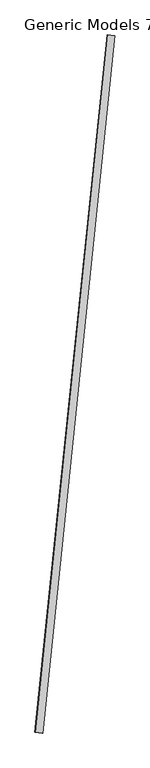
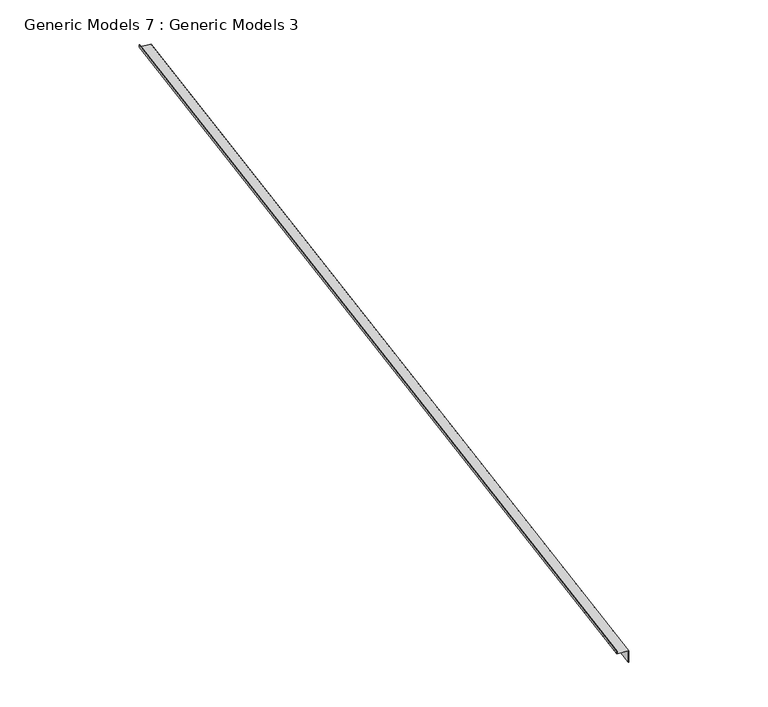
"""IFC4 building model written with IfcOpenShell, lengths in millimetres: proxy geometry, Generic Models 7 : Generic Models 3."""

import ifcopenshell
import ifcopenshell.guid

model = None  # the IFC model being written
_history = None  # IfcOwnerHistory: only IFC2X3 demands one
_inside = {}  # id of a spatial element -> (the spatial element, [elements in it])
_under = {}  # id of a project, library or spatial element -> (it, [spatial elements below it])
_declared = {}  # id of a project -> (the project, [libraries it declares])
_typed = {}  # id of a type object -> (the type object, [elements of that type])
_made_of = {}  # id of a material, layer set ... -> (it, [elements and type objects made of it])


def new_model(schema):
    """Start an empty IFC model of exactly this schema.

    Asked for "IFC4X3", IfcOpenShell would pick the latest addendum, in which some entities
    have other attributes; the version numbers below select the first issue.
    IFC2X3 requires an IfcOwnerHistory on every rooted entity: one is made here for all.
    """
    global model, _history
    if schema == "IFC4X3":
        model = ifcopenshell.file(schema_version=(4, 3, 0, 0))
    else:
        model = ifcopenshell.file(schema=schema)
    _inside.clear()
    _under.clear()
    _declared.clear()
    _typed.clear()
    _made_of.clear()
    _history = None
    if model.schema == "IFC2X3":
        org = make("IfcOrganization", Name="unknown")
        user = make(
            "IfcPersonAndOrganization",
            ThePerson=make("IfcPerson", FamilyName="unknown"),
            TheOrganization=org,
        )
        app = make(
            "IfcApplication",
            ApplicationDeveloper=org,
            Version="unknown",
            ApplicationFullName="unknown",
            ApplicationIdentifier="unknown",
        )
        _history = make(
            "IfcOwnerHistory",
            OwningUser=user,
            OwningApplication=app,
            ChangeAction="ADDED",
            CreationDate=0,
        )
    return model


def make(cls, **values):
    """One entity of the class cls with the attributes given. An attribute that is None is left unset."""
    return model.create_entity(
        cls, **{name: value for name, value in values.items() if value is not None}
    )


def rooted(cls, **values):
    """An entity with a GlobalId (a new one), such as an element, a storey or a relation."""
    return make(cls, GlobalId=ifcopenshell.guid.new(), OwnerHistory=_history, **values)


def si_unit(unit_type, name, prefix=None):
    """IfcSIUnit, for example si_unit("LENGTHUNIT", "METRE", prefix="MILLI")."""
    return make("IfcSIUnit", UnitType=unit_type, Prefix=prefix, Name=name)


def assignment(units):
    """IfcUnitAssignment: the units of a project."""
    return None if units is None else make("IfcUnitAssignment", Units=units)


def point(xyz):
    """IfcCartesianPoint."""
    return None if xyz is None else make("IfcCartesianPoint", Coordinates=xyz)


def direction(xyz):
    """IfcDirection."""
    return None if xyz is None else make("IfcDirection", DirectionRatios=xyz)


def frame(location, z_axis=None, x_axis=None):
    """IfcAxis2Placement3D, a coordinate frame: its origin and axes. An axis left out is left unset."""
    return make(
        "IfcAxis2Placement3D",
        Location=point(location),
        Axis=direction(z_axis),
        RefDirection=direction(x_axis),
    )


def origin():
    """The frame at (0, 0, 0) with its axes left unset."""
    return frame((0.0, 0.0, 0.0))


def place(relative_to, where):
    """IfcLocalPlacement: puts the frame where relative to a parent placement (None: the world)."""
    return make(
        "IfcLocalPlacement", PlacementRelTo=relative_to, RelativePlacement=where
    )


def context(
    kind, dimensions, precision=None, world=None, true_north=None, identifier=None
):
    """IfcGeometricRepresentationContext, for example the 3D "Model" context."""
    return make(
        "IfcGeometricRepresentationContext",
        ContextIdentifier=identifier,
        ContextType=kind,
        CoordinateSpaceDimension=dimensions,
        Precision=precision,
        WorldCoordinateSystem=world,
        TrueNorth=true_north,
    )


def project(units=None, contexts=None):
    """IfcProject with its units and contexts."""
    return rooted(
        "IfcProject",
        Name="project",
        RepresentationContexts=contexts,
        UnitsInContext=assignment(units),
    )


def spatial(cls, under=None, at=None, **own):
    """A site, building, storey or space (cls), placed at a placement, below another one or the project."""
    s = rooted(cls, ObjectPlacement=at, **own)
    if under is not None:
        _under.setdefault(under.id(), (under, []))[1].append(s)
    return s


def polyline(points):
    """IfcPolyline through the points."""
    return make("IfcPolyline", Points=[point(p) for p in points])


def outline(outer, holes=None, kind="AREA"):
    """IfcArbitraryClosedProfileDef: a profile drawn as a closed curve; with holes, ...WithVoids."""
    if holes is None:
        return make("IfcArbitraryClosedProfileDef", ProfileType=kind, OuterCurve=outer)
    return make(
        "IfcArbitraryProfileDefWithVoids",
        ProfileType=kind,
        OuterCurve=outer,
        InnerCurves=holes,
    )


def extrude(swept, where, along, depth):
    """IfcExtrudedAreaSolid: the profile swept, set in the frame where, extruded along a direction by depth."""
    return make(
        "IfcExtrudedAreaSolid",
        SweptArea=swept,
        Position=where,
        ExtrudedDirection=direction(along),
        Depth=depth,
    )


def shape(context_of_items, identifier, shape_type, items):
    """IfcShapeRepresentation: the items that make up one representation, for example the "Body"."""
    return make(
        "IfcShapeRepresentation",
        ContextOfItems=context_of_items,
        RepresentationIdentifier=identifier,
        RepresentationType=shape_type,
        Items=items,
    )


def source(mapping_origin, context_of_items, identifier, shape_type, items):
    """IfcRepresentationMap: a shape defined once, which mapped items show again and again."""
    return make(
        "IfcRepresentationMap",
        MappingOrigin=mapping_origin,
        MappedRepresentation=shape(context_of_items, identifier, shape_type, items),
    )


def transform(
    local_origin,
    x_axis=None,
    y_axis=None,
    z_axis=None,
    scale=None,
    scale2=None,
    scale3=None,
    uniform=True,
):
    """IfcCartesianTransformationOperator3D, or its non-uniform kind. x_axis, y_axis, z_axis: its Axis1, 2, 3."""
    if uniform:
        return make(
            "IfcCartesianTransformationOperator3D",
            Axis1=direction(x_axis),
            Axis2=direction(y_axis),
            LocalOrigin=point(local_origin),
            Scale=scale,
            Axis3=direction(z_axis),
        )
    return make(
        "IfcCartesianTransformationOperator3DnonUniform",
        Axis1=direction(x_axis),
        Axis2=direction(y_axis),
        LocalOrigin=point(local_origin),
        Scale=scale,
        Axis3=direction(z_axis),
        Scale2=scale2,
        Scale3=scale3,
    )


def mapped(mapping_source, mapping_target):
    """IfcMappedItem: shows the shape of a source again, moved by a transform."""
    return make(
        "IfcMappedItem", MappingSource=mapping_source, MappingTarget=mapping_target
    )


def made_of(thing, what):
    """Note that an element or type object is made of a material, layer set ...; save() writes the relation."""
    if what is not None:
        _made_of.setdefault(what.id(), (what, []))[1].append(thing)
    return thing


def element(
    cls,
    number,
    at=None,
    inside=None,
    cuts=None,
    type_object=None,
    material=None,
    context=None,
    identifier="Body",
    shape_type=None,
    held_by="IfcProductDefinitionShape",
    body=None,
    shapes=None,
    **own,
):
    """One element of the class cls, such as IfcWall. Its Tag is "e" and its number.

    at: its placement. inside: the storey or other place that contains it. cuts: it is an
    opening in that element (IfcRelVoidsElement). A single representation is given by context,
    identifier, shape_type and body (its items); several are given by shapes. held_by: the class
    of the entity that holds the representations. save() writes the other relations.
    """
    e = rooted(cls, Tag="e%d" % number, ObjectPlacement=at, **own)
    if body is not None:
        shapes = [shape(context, identifier, shape_type, body)]
    if shapes is not None:
        e.Representation = make(held_by, Representations=shapes)
    if inside is not None:
        _inside.setdefault(inside.id(), (inside, []))[1].append(e)
    if cuts is not None:
        rooted(
            "IfcRelVoidsElement", RelatingBuildingElement=cuts, RelatedOpeningElement=e
        )
    if type_object is not None:
        _typed.setdefault(type_object.id(), (type_object, []))[1].append(e)
    return made_of(e, material)


def aggregate(whole, parts):
    """IfcRelAggregates: a whole, such as a stair, and the parts it consists of."""
    return rooted("IfcRelAggregates", RelatingObject=whole, RelatedObjects=parts)


def save(model, path):
    """Write the relations noted so far, then the file.

    IfcRelAggregates (storeys below a building ...), IfcRelContainedInSpatialStructure (elements
    in a storey), IfcRelDefinesByType, IfcRelAssociatesMaterial and IfcRelDeclares: one each for
    every whole, place, type object, material and project.
    """
    for whole, parts in _under.values():
        aggregate(whole, parts)
    for where, things in _inside.values():
        rooted(
            "IfcRelContainedInSpatialStructure",
            RelatedElements=things,
            RelatingStructure=where,
        )
    for kind, things in _typed.values():
        rooted("IfcRelDefinesByType", RelatedObjects=things, RelatingType=kind)
    for what, things in _made_of.values():
        rooted("IfcRelAssociatesMaterial", RelatedObjects=things, RelatingMaterial=what)
    for by, libraries in _declared.values():
        rooted("IfcRelDeclares", RelatingContext=by, RelatedDefinitions=libraries)
    model.write(path)


def generic_models_7_generic_models_3_f2663baf(model_context):
    return source(origin(), model_context, "Body", "SweptSolid", [
        extrude(outline(polyline([(0.0, 0.0), (0.0, -63.5), (-1.5875001, -63.5), (-1.5875, -1.5875), (-58.7375, -1.5875), (-58.7375, 12.6998049), (-57.1500001, 12.699805), (-57.1500001, 0.0), (0.0, 0.0)])), frame((34321.9394407, 30911.0576425, 271782.5299467), z_axis=(-0.10293344407674772, -0.9946674410191906, 0.006433340254794664), x_axis=(0.9946880183641726, -0.1029356401670686, -1.030297607946377e-05)), (0.0, 0.0, 1.0), 5311.9304914),
    ])


if __name__ == "__main__":
    model = new_model("IFC4")
    model_context = context("Model", 3, world=origin())
    ifc_project = project(units=[si_unit("LENGTHUNIT", "METRE", prefix="MILLI")], contexts=[model_context])
    site = spatial("IfcSite", under=ifc_project)
    building = spatial("IfcBuilding", under=site)
    placement = place(None, origin())
    generic_models_7_generic_models_3_shape = generic_models_7_generic_models_3_f2663baf(model_context)
    element("IfcBuildingElementProxy", 1, Name="Generic Models 7 : Generic Models 3", ObjectType="Generic Models 7 : Generic Models 3", at=placement, inside=building, context=model_context, shape_type="MappedRepresentation", body=[
        mapped(generic_models_7_generic_models_3_shape, transform((0.0, 0.0, 0.0), x_axis=(1.0, 0.0, 0.0), y_axis=(0.0, 1.0, 0.0), z_axis=(0.0, 0.0, 1.0))),
    ])
    save(model, "model.ifc")

# Revit data of these elements
# Element 1 (IfcBuildingElementProxy, "Generic Models 7 : Generic Models 3")
#   Materials on its faces: "GALV. BRAKE METAL - (COLOR: MATCH ALUM. WINDOWS)"
# Materials
#   "GALV. BRAKE METAL - (COLOR: MATCH ALUM. WINDOWS)": class "Generic", colour RGB 234 234 234, transparency 0, Cost = 0
